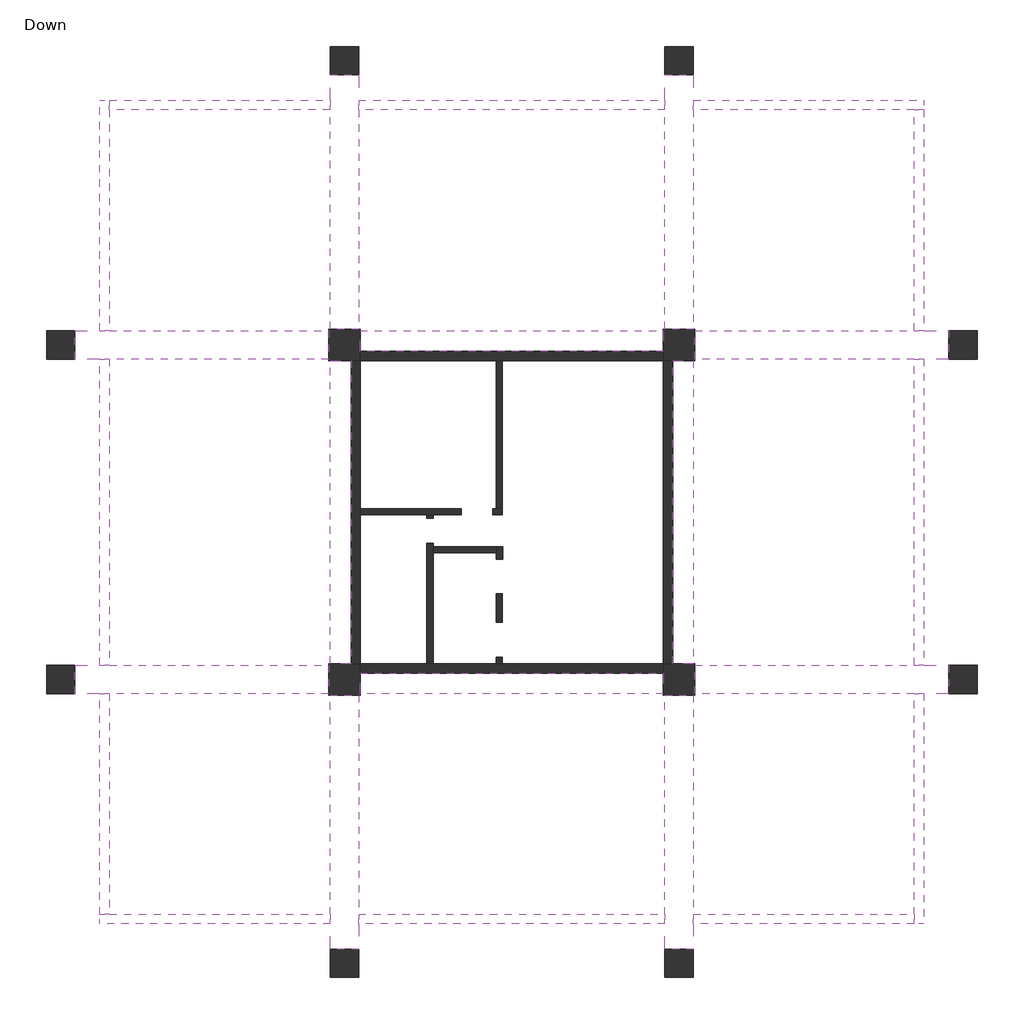
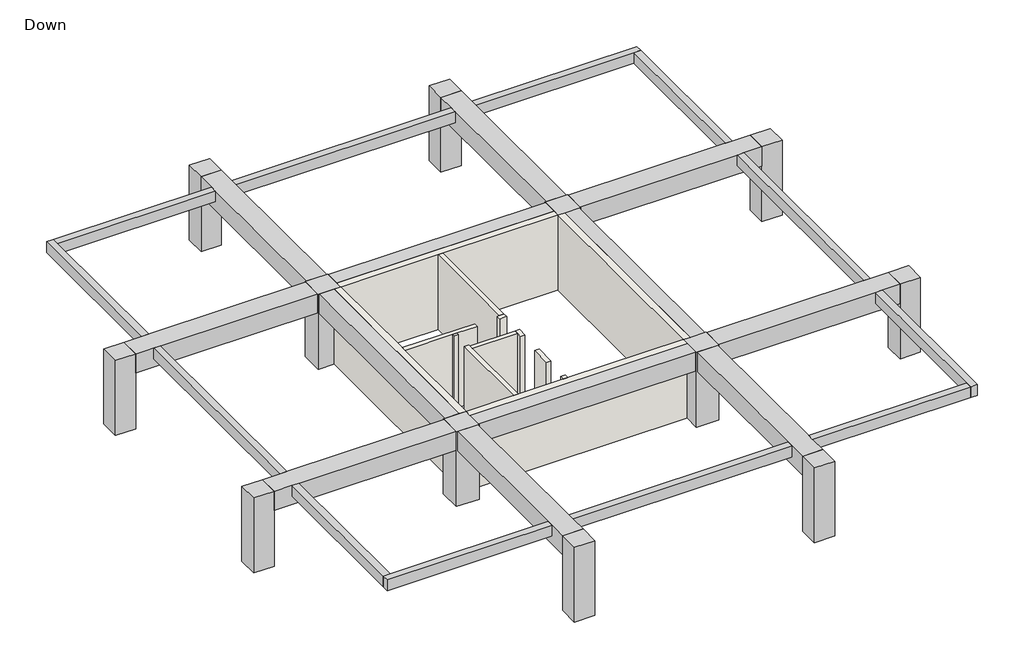
# One storey: 24 beams, 13 walls, 12 columns.
"""IFC4 building model written with IfcOpenShell, lengths in millimetres."""

import ifcopenshell
import ifcopenshell.guid

model = None  # the IFC model being written
_history = None  # IfcOwnerHistory: only IFC2X3 demands one
_inside = {}  # id of a spatial element -> (the spatial element, [elements in it])
_under = {}  # id of a project, library or spatial element -> (it, [spatial elements below it])
_declared = {}  # id of a project -> (the project, [libraries it declares])
_typed = {}  # id of a type object -> (the type object, [elements of that type])
_made_of = {}  # id of a material, layer set ... -> (it, [elements and type objects made of it])


def new_model(schema):
    """Start an empty IFC model of exactly this schema.

    Asked for "IFC4X3", IfcOpenShell would pick the latest addendum, in which some entities
    have other attributes; the version numbers below select the first issue.
    IFC2X3 requires an IfcOwnerHistory on every rooted entity: one is made here for all.
    """
    global model, _history
    if schema == "IFC4X3":
        model = ifcopenshell.file(schema_version=(4, 3, 0, 0))
    else:
        model = ifcopenshell.file(schema=schema)
    _inside.clear()
    _under.clear()
    _declared.clear()
    _typed.clear()
    _made_of.clear()
    _history = None
    if model.schema == "IFC2X3":
        org = make("IfcOrganization", Name="unknown")
        user = make(
            "IfcPersonAndOrganization",
            ThePerson=make("IfcPerson", FamilyName="unknown"),
            TheOrganization=org,
        )
        app = make(
            "IfcApplication",
            ApplicationDeveloper=org,
            Version="unknown",
            ApplicationFullName="unknown",
            ApplicationIdentifier="unknown",
        )
        _history = make(
            "IfcOwnerHistory",
            OwningUser=user,
            OwningApplication=app,
            ChangeAction="ADDED",
            CreationDate=0,
        )
    return model


def make(cls, **values):
    """One entity of the class cls with the attributes given. An attribute that is None is left unset."""
    return model.create_entity(
        cls, **{name: value for name, value in values.items() if value is not None}
    )


def rooted(cls, **values):
    """An entity with a GlobalId (a new one), such as an element, a storey or a relation."""
    return make(cls, GlobalId=ifcopenshell.guid.new(), OwnerHistory=_history, **values)


def si_unit(unit_type, name, prefix=None):
    """IfcSIUnit, for example si_unit("LENGTHUNIT", "METRE", prefix="MILLI")."""
    return make("IfcSIUnit", UnitType=unit_type, Prefix=prefix, Name=name)


def assignment(units):
    """IfcUnitAssignment: the units of a project."""
    return None if units is None else make("IfcUnitAssignment", Units=units)


def point(xyz):
    """IfcCartesianPoint."""
    return None if xyz is None else make("IfcCartesianPoint", Coordinates=xyz)


def direction(xyz):
    """IfcDirection."""
    return None if xyz is None else make("IfcDirection", DirectionRatios=xyz)


def frame(location, z_axis=None, x_axis=None):
    """IfcAxis2Placement3D, a coordinate frame: its origin and axes. An axis left out is left unset."""
    return make(
        "IfcAxis2Placement3D",
        Location=point(location),
        Axis=direction(z_axis),
        RefDirection=direction(x_axis),
    )


def origin():
    """The frame at (0, 0, 0) with its axes left unset."""
    return frame((0.0, 0.0, 0.0))


def origin_with_axes():
    """The frame at (0, 0, 0) with the z axis (0, 0, 1) and the x axis (1, 0, 0) written out."""
    return frame((0.0, 0.0, 0.0), z_axis=(0.0, 0.0, 1.0), x_axis=(1.0, 0.0, 0.0))


def place(relative_to, where):
    """IfcLocalPlacement: puts the frame where relative to a parent placement (None: the world)."""
    return make(
        "IfcLocalPlacement", PlacementRelTo=relative_to, RelativePlacement=where
    )


def context(
    kind, dimensions, precision=None, world=None, true_north=None, identifier=None
):
    """IfcGeometricRepresentationContext, for example the 3D "Model" context."""
    return make(
        "IfcGeometricRepresentationContext",
        ContextIdentifier=identifier,
        ContextType=kind,
        CoordinateSpaceDimension=dimensions,
        Precision=precision,
        WorldCoordinateSystem=world,
        TrueNorth=true_north,
    )


def project(units=None, contexts=None):
    """IfcProject with its units and contexts."""
    return rooted(
        "IfcProject",
        Name="project",
        RepresentationContexts=contexts,
        UnitsInContext=assignment(units),
    )


def spatial(cls, under=None, at=None, **own):
    """A site, building, storey or space (cls), placed at a placement, below another one or the project."""
    s = rooted(cls, ObjectPlacement=at, **own)
    if under is not None:
        _under.setdefault(under.id(), (under, []))[1].append(s)
    return s


def polyline(points):
    """IfcPolyline through the points."""
    return make("IfcPolyline", Points=[point(p) for p in points])


def outline(outer, holes=None, kind="AREA"):
    """IfcArbitraryClosedProfileDef: a profile drawn as a closed curve; with holes, ...WithVoids."""
    if holes is None:
        return make("IfcArbitraryClosedProfileDef", ProfileType=kind, OuterCurve=outer)
    return make(
        "IfcArbitraryProfileDefWithVoids",
        ProfileType=kind,
        OuterCurve=outer,
        InnerCurves=holes,
    )


def extrude(swept, where, along, depth):
    """IfcExtrudedAreaSolid: the profile swept, set in the frame where, extruded along a direction by depth."""
    return make(
        "IfcExtrudedAreaSolid",
        SweptArea=swept,
        Position=where,
        ExtrudedDirection=direction(along),
        Depth=depth,
    )


def faces_of(points, faces, orient=None, outer=None):
    """IfcFace entities. A face is a list of loops; a loop is a list of indices into points, from 0.

    orient and outer hold one flag for each loop. By default every Orientation is true, the
    first loop of a face is its IfcFaceOuterBound and the others are IfcFaceBound.
    """
    made = []
    for i, loops in enumerate(faces):
        bounds = []
        for j, loop in enumerate(loops):
            is_outer = j == 0 if outer is None else outer[i][j]
            bounds.append(
                make(
                    "IfcFaceOuterBound" if is_outer else "IfcFaceBound",
                    Bound=make("IfcPolyLoop", Polygon=[points[k] for k in loop]),
                    Orientation=True if orient is None else orient[i][j],
                )
            )
        made.append(make("IfcFace", Bounds=bounds))
    return made


def faceted_brep(points, faces, orient=None, outer=None, voids=None):
    """IfcFacetedBrep: a solid bounded by flat faces; with voids (closed shells), ...WithVoids."""
    shared = [point(p) for p in points]
    hull = make("IfcClosedShell", CfsFaces=faces_of(shared, faces, orient, outer))
    if voids is None:
        return make("IfcFacetedBrep", Outer=hull)
    return make(
        "IfcFacetedBrepWithVoids",
        Outer=hull,
        Voids=[
            make(cls, CfsFaces=faces_of(shared, fs, o, b)) for cls, fs, o, b in voids
        ],
    )


def shape(context_of_items, identifier, shape_type, items):
    """IfcShapeRepresentation: the items that make up one representation, for example the "Body"."""
    return make(
        "IfcShapeRepresentation",
        ContextOfItems=context_of_items,
        RepresentationIdentifier=identifier,
        RepresentationType=shape_type,
        Items=items,
    )


def made_of(thing, what):
    """Note that an element or type object is made of a material, layer set ...; save() writes the relation."""
    if what is not None:
        _made_of.setdefault(what.id(), (what, []))[1].append(thing)
    return thing


def element(
    cls,
    number,
    at=None,
    inside=None,
    cuts=None,
    type_object=None,
    material=None,
    context=None,
    identifier="Body",
    shape_type=None,
    held_by="IfcProductDefinitionShape",
    body=None,
    shapes=None,
    **own,
):
    """One element of the class cls, such as IfcWall. Its Tag is "e" and its number.

    at: its placement. inside: the storey or other place that contains it. cuts: it is an
    opening in that element (IfcRelVoidsElement). A single representation is given by context,
    identifier, shape_type and body (its items); several are given by shapes. held_by: the class
    of the entity that holds the representations. save() writes the other relations.
    """
    e = rooted(cls, Tag="e%d" % number, ObjectPlacement=at, **own)
    if body is not None:
        shapes = [shape(context, identifier, shape_type, body)]
    if shapes is not None:
        e.Representation = make(held_by, Representations=shapes)
    if inside is not None:
        _inside.setdefault(inside.id(), (inside, []))[1].append(e)
    if cuts is not None:
        rooted(
            "IfcRelVoidsElement", RelatingBuildingElement=cuts, RelatedOpeningElement=e
        )
    if type_object is not None:
        _typed.setdefault(type_object.id(), (type_object, []))[1].append(e)
    return made_of(e, material)


def aggregate(whole, parts):
    """IfcRelAggregates: a whole, such as a stair, and the parts it consists of."""
    return rooted("IfcRelAggregates", RelatingObject=whole, RelatedObjects=parts)


def save(model, path):
    """Write the relations noted so far, then the file.

    IfcRelAggregates (storeys below a building ...), IfcRelContainedInSpatialStructure (elements
    in a storey), IfcRelDefinesByType, IfcRelAssociatesMaterial and IfcRelDeclares: one each for
    every whole, place, type object, material and project.
    """
    for whole, parts in _under.values():
        aggregate(whole, parts)
    for where, things in _inside.values():
        rooted(
            "IfcRelContainedInSpatialStructure",
            RelatedElements=things,
            RelatingStructure=where,
        )
    for kind, things in _typed.values():
        rooted("IfcRelDefinesByType", RelatedObjects=things, RelatingType=kind)
    for what, things in _made_of.values():
        rooted("IfcRelAssociatesMaterial", RelatedObjects=things, RelatingMaterial=what)
    for by, libraries in _declared.values():
        rooted("IfcRelDeclares", RelatingContext=by, RelatedDefinitions=libraries)
    model.write(path)


model = new_model("IFC4")

# Units and contexts
model_context = context("Model", 3, world=origin())
ifc_project = project(units=[si_unit("LENGTHUNIT", "METRE", prefix="MILLI")], contexts=[model_context])

# Site, building, storey
site = spatial("IfcSite", under=ifc_project)
building = spatial("IfcBuilding", under=site)
storey = spatial("IfcBuildingStorey", under=building, Name="Down", Elevation=0.0)

# Beams
placement = place(None, origin())
element("IfcBeam", 1, ObjectType="Concrete Rectengular Beam : 30/50", at=placement, inside=storey, context=model_context, shape_type="Brep", body=[
    faceted_brep([(-5980.9538985, 16952.588413, 3500.0), (-5980.9538985, 17252.588413, 3500.0), (-15690.3344173, 17252.588413, 3500.0), (-15690.3344173, 16952.588413, 3500.0), (-5980.9538985, 16952.588413, 3000.0), (-5980.9538985, 16952.588413, 3250.0), (-15690.3344173, 16952.588413, 3250.0), (-15690.3344173, 16952.588413, 3000.0), (-5980.9538985, 17252.588413, 3000.0), (-15690.3344173, 17252.588413, 3000.0)], [[[0, 1, 2, 3]], [[4, 5, 0, 3, 6, 7]], [[8, 4, 7, 9]], [[1, 8, 9, 2]], [[1, 0, 5, 4, 8]], [[3, 2, 9, 7, 6]]]),
])
element("IfcBeam", 2, ObjectType="Concrete Rectengular Beam : 30/50", at=placement, inside=storey, context=model_context, shape_type="Brep", body=[
    faceted_brep([(2219.0461015, 16952.588413, 3500.0), (2219.0461015, 17252.588413, 3500.0), (-5080.9538985, 17252.588413, 3500.0), (-5080.9538985, 16952.588413, 3500.0), (1919.0461015, 16952.588413, 3500.0), (2219.0461015, 16952.588413, 3000.0), (-5080.9538985, 16952.588413, 3250.0), (-5080.9538985, 16952.588413, 3000.0), (1919.0461015, 16952.588413, 3000.0), (2219.0461015, 17252.588413, 3000.0), (-5080.9538985, 17252.588413, 3000.0)], [[[0, 1, 2, 3, 4]], [[5, 0, 4, 3, 6, 7, 8]], [[9, 5, 8, 7, 10]], [[1, 9, 10, 2]], [[3, 2, 10, 7, 6]], [[1, 0, 5, 9]]]),
])
element("IfcBeam", 3, ObjectType="Concrete Rectengular Beam : 30/50", at=placement, inside=storey, context=model_context, shape_type="Brep", body=[
    faceted_brep([(2219.0461015, 16952.588413, 3500.0), (1919.0461015, 16952.588413, 3500.0), (1919.0461015, 9953.1817285, 3500.0), (2219.0461015, 9953.1817285, 3500.0), (1919.0461015, 16952.588413, 3250.0), (1919.0461015, 16952.588413, 3000.0), (1919.0461015, 9953.1817285, 3000.0), (1919.0461015, 9953.1817285, 3250.0), (2219.0461015, 16952.588413, 3000.0), (2219.0461015, 9953.1817285, 3000.0)], [[[0, 1, 2, 3]], [[1, 4, 5, 6, 7, 2]], [[5, 8, 9, 6]], [[8, 0, 3, 9]], [[1, 0, 8, 5, 4]], [[3, 2, 7, 6, 9]]]),
])
element("IfcBeam", 4, ObjectType="Concrete Rectengular Beam : 30/50", at=placement, inside=storey, context=model_context, shape_type="Brep", body=[
    faceted_brep([(2219.0461015, 9053.1817285, 3500.0), (1919.0461015, 9053.1817285, 3500.0), (1919.0461015, -648.2491126, 3500.0), (2219.0461015, -648.2491126, 3500.0), (1919.0461015, 9053.1817285, 3250.0), (1919.0461015, 9053.1817285, 3000.0), (1919.0461015, -648.2491126, 3000.0), (1919.0461015, -648.2491126, 3250.0), (2219.0461015, 9053.1817285, 3000.0), (2219.0461015, -648.2491126, 3000.0)], [[[0, 1, 2, 3]], [[1, 4, 5, 6, 7, 2]], [[5, 8, 9, 6]], [[8, 0, 3, 9]], [[1, 0, 8, 5, 4]], [[3, 2, 7, 6, 9]]]),
])
element("IfcBeam", 5, ObjectType="Concrete Rectengular Beam : 30/50", at=placement, inside=storey, context=model_context, shape_type="Brep", body=[
    faceted_brep([(1919.0461015, -8848.2491126, 3500.0), (2219.0461015, -8848.2491126, 3500.0), (2219.0461015, -1548.2491126, 3500.0), (1919.0461015, -1548.2491126, 3500.0), (1919.0461015, -8548.2491126, 3500.0), (1919.0461015, -8848.2491126, 3000.0), (1919.0461015, -1548.2491126, 3250.0), (1919.0461015, -1548.2491126, 3000.0), (1919.0461015, -8548.2491126, 3000.0), (2219.0461015, -8848.2491126, 3000.0), (2219.0461015, -1548.2491126, 3000.0)], [[[0, 1, 2, 3, 4]], [[5, 0, 4, 3, 6, 7, 8]], [[9, 5, 8, 7, 10]], [[1, 9, 10, 2]], [[3, 2, 10, 7, 6]], [[1, 0, 5, 9]]]),
])
element("IfcBeam", 6, ObjectType="Concrete Rectengular Beam : 30/50", at=placement, inside=storey, context=model_context, shape_type="Brep", body=[
    faceted_brep([(1919.0461015, -8848.2491126, 3500.0), (1919.0461015, -8548.2491126, 3500.0), (-5080.9538985, -8548.2491126, 3500.0), (-5080.9538985, -8848.2491126, 3500.0), (1919.0461015, -8548.2491126, 3250.0), (1919.0461015, -8548.2491126, 3000.0), (-5080.9538985, -8548.2491126, 3000.0), (-5080.9538985, -8548.2491126, 3250.0), (1919.0461015, -8848.2491126, 3000.0), (-5080.9538985, -8848.2491126, 3000.0)], [[[0, 1, 2, 3]], [[1, 4, 5, 6, 7, 2]], [[5, 8, 9, 6]], [[8, 0, 3, 9]], [[1, 0, 8, 5, 4]], [[3, 2, 7, 6, 9]]]),
])
element("IfcBeam", 7, ObjectType="Concrete Rectengular Beam : 30/50", at=placement, inside=storey, context=model_context, shape_type="Brep", body=[
    faceted_brep([(-15690.3344173, -8548.2491126, 3500.0), (-15690.3344173, -8848.2491126, 3500.0), (-5980.9538985, -8848.2491126, 3500.0), (-5980.9538985, -8548.2491126, 3500.0), (-15690.3344173, -8548.2491126, 3000.0), (-15690.3344173, -8548.2491126, 3250.0), (-5980.9538985, -8548.2491126, 3250.0), (-5980.9538985, -8548.2491126, 3000.0), (-15690.3344173, -8848.2491126, 3000.0), (-5980.9538985, -8848.2491126, 3000.0)], [[[0, 1, 2, 3]], [[4, 5, 0, 3, 6, 7]], [[8, 4, 7, 9]], [[1, 8, 9, 2]], [[1, 0, 5, 4, 8]], [[3, 2, 9, 7, 6]]]),
])
element("IfcBeam", 8, ObjectType="Concrete Rectengular Beam : 30/50", at=placement, inside=storey, context=model_context, shape_type="Brep", body=[
    faceted_brep([(-23890.3344173, -8548.2491126, 3500.0), (-23890.3344173, -8848.2491126, 3500.0), (-16590.3344173, -8848.2491126, 3500.0), (-16590.3344173, -8548.2491126, 3500.0), (-23590.3344173, -8548.2491126, 3500.0), (-23890.3344173, -8548.2491126, 3000.0), (-16590.3344173, -8548.2491126, 3250.0), (-16590.3344173, -8548.2491126, 3000.0), (-23590.3344173, -8548.2491126, 3000.0), (-23890.3344173, -8848.2491126, 3000.0), (-16590.3344173, -8848.2491126, 3000.0)], [[[0, 1, 2, 3, 4]], [[5, 0, 4, 3, 6, 7, 8]], [[9, 5, 8, 7, 10]], [[1, 9, 10, 2]], [[3, 2, 10, 7, 6]], [[1, 0, 5, 9]]]),
])
element("IfcBeam", 9, ObjectType="Concrete Rectengular Beam : 30/50", at=placement, inside=storey, context=model_context, shape_type="Brep", body=[
    faceted_brep([(-23890.3344173, -8548.2491126, 3500.0), (-23590.3344173, -8548.2491126, 3500.0), (-23590.3344173, -1548.2491126, 3500.0), (-23890.3344173, -1548.2491126, 3500.0), (-23590.3344173, -8548.2491126, 3250.0), (-23590.3344173, -8548.2491126, 3000.0), (-23590.3344173, -1548.2491126, 3000.0), (-23590.3344173, -1548.2491126, 3250.0), (-23890.3344173, -8548.2491126, 3000.0), (-23890.3344173, -1548.2491126, 3000.0)], [[[0, 1, 2, 3]], [[1, 4, 5, 6, 7, 2]], [[5, 8, 9, 6]], [[8, 0, 3, 9]], [[1, 0, 8, 5, 4]], [[3, 2, 7, 6, 9]]]),
])
element("IfcBeam", 10, ObjectType="Concrete Rectengular Beam : 30/50", at=placement, inside=storey, context=model_context, shape_type="Brep", body=[
    faceted_brep([(-23590.3344173, 9053.1817285, 3500.0), (-23890.3344173, 9053.1817285, 3500.0), (-23890.3344173, -648.2491126, 3500.0), (-23590.3344173, -648.2491126, 3500.0), (-23590.3344173, 9053.1817285, 3000.0), (-23590.3344173, 9053.1817285, 3250.0), (-23590.3344173, -648.2491126, 3250.0), (-23590.3344173, -648.2491126, 3000.0), (-23890.3344173, 9053.1817285, 3000.0), (-23890.3344173, -648.2491126, 3000.0)], [[[0, 1, 2, 3]], [[4, 5, 0, 3, 6, 7]], [[8, 4, 7, 9]], [[1, 8, 9, 2]], [[1, 0, 5, 4, 8]], [[3, 2, 9, 7, 6]]]),
])
element("IfcBeam", 11, ObjectType="Concrete Rectengular Beam : 30/50", at=placement, inside=storey, context=model_context, shape_type="Brep", body=[
    faceted_brep([(-23590.3344173, 17253.1817285, 3500.0), (-23890.3344173, 17253.1817285, 3500.0), (-23890.3344173, 9953.1817285, 3500.0), (-23590.3344173, 9953.1817285, 3500.0), (-23590.3344173, 16953.1817285, 3500.0), (-23590.3344173, 17253.1817285, 3000.0), (-23590.3344173, 9953.1817285, 3250.0), (-23590.3344173, 9953.1817285, 3000.0), (-23590.3344173, 16953.1817285, 3000.0), (-23890.3344173, 17253.1817285, 3000.0), (-23890.3344173, 9953.1817285, 3000.0)], [[[0, 1, 2, 3, 4]], [[5, 0, 4, 3, 6, 7, 8]], [[9, 5, 8, 7, 10]], [[1, 9, 10, 2]], [[3, 2, 10, 7, 6]], [[1, 0, 5, 9]]]),
])
element("IfcBeam", 12, ObjectType="Concrete Rectengular Beam : 30/50", at=placement, inside=storey, context=model_context, shape_type="Brep", body=[
    faceted_brep([(-23590.3344173, 17253.1817285, 3500.0), (-23590.3344173, 16953.1817285, 3500.0), (-16590.3344173, 16953.1817285, 3500.0), (-16590.3344173, 17253.1817285, 3500.0), (-23590.3344173, 16953.1817285, 3250.0), (-23590.3344173, 16953.1817285, 3000.0), (-16590.3344173, 16953.1817285, 3000.0), (-16590.3344173, 16953.1817285, 3250.0), (-23590.3344173, 17253.1817285, 3000.0), (-16590.3344173, 17253.1817285, 3000.0)], [[[0, 1, 2, 3]], [[1, 4, 5, 6, 7, 2]], [[5, 8, 9, 6]], [[8, 0, 3, 9]], [[1, 0, 8, 5, 4]], [[3, 2, 7, 6, 9]]]),
])
element("IfcBeam", 13, ObjectType="Concrete Rectengular Beam : 90/90", at=placement, inside=storey, context=model_context, shape_type="Brep", body=[
    faceted_brep([(3013.7426277, 9053.1817285, 3500.0), (3013.7426277, 9953.1817285, 3500.0), (2219.0461015, 9953.1817285, 3500.0), (1919.0461015, 9953.1817285, 3500.0), (-5030.9538985, 9953.1817285, 3500.0), (-5030.9538985, 9053.1817285, 3500.0), (1919.0461015, 9053.1817285, 3500.0), (2219.0461015, 9053.1817285, 3500.0), (3013.7426277, 9953.1817285, 2600.0), (-5030.9538985, 9953.1817285, 2600.0), (-5030.9538985, 9953.1817285, 3250.0), (3013.7426277, 9053.1817285, 2600.0), (-5030.9538985, 9053.1817285, 2600.0), (-5030.9538985, 9053.1817285, 3250.0)], [[[0, 1, 2, 3, 4, 5, 6, 7]], [[1, 8, 9, 10, 4, 3, 2]], [[8, 11, 12, 9]], [[11, 0, 7, 6, 5, 13, 12]], [[1, 0, 11, 8]], [[5, 4, 10, 9, 12, 13]]]),
])
element("IfcBeam", 14, ObjectType="Concrete Rectengular Beam : 90/90", at=placement, inside=storey, context=model_context, shape_type="Brep", body=[
    faceted_brep([(-6030.9538985, 9953.1817285, 3500.0), (-15640.3344173, 9953.1817285, 3500.0), (-15640.3344173, 9303.1817285, 3500.0), (-6030.9538985, 9303.1817285, 3500.0), (-15640.3344173, 9953.1817285, 2600.0), (-15640.3344173, 9953.1817285, 3250.0), (-6030.9538985, 9953.1817285, 3250.0), (-6030.9538985, 9953.1817285, 2600.0), (-6030.9538985, 9303.1817285, 2600.0), (-15640.3344173, 9303.1817285, 2600.0)], [[[0, 1, 2, 3]], [[4, 5, 1, 0, 6, 7]], [[4, 7, 8, 9]], [[1, 5, 4, 9, 2]], [[7, 6, 0, 3, 8]], [[3, 2, 9, 8]]]),
])
element("IfcBeam", 15, ObjectType="Concrete Rectengular Beam : 90/90", at=placement, inside=storey, context=model_context, shape_type="Brep", body=[
    faceted_brep([(-24681.3411297, 9953.1817285, 3500.0), (-24681.3411297, 9053.1817285, 3500.0), (-23890.3344173, 9053.1817285, 3500.0), (-23590.3344173, 9053.1817285, 3500.0), (-16640.3344173, 9053.1817285, 3500.0), (-16640.3344173, 9953.1817285, 3500.0), (-23590.3344173, 9953.1817285, 3500.0), (-23890.3344173, 9953.1817285, 3500.0), (-24681.3411297, 9953.1817285, 2600.0), (-16640.3344173, 9953.1817285, 3250.0), (-16640.3344173, 9953.1817285, 2600.0), (-24681.3411297, 9053.1817285, 2600.0), (-16640.3344173, 9053.1817285, 2600.0), (-16640.3344173, 9053.1817285, 3250.0)], [[[0, 1, 2, 3, 4, 5, 6, 7]], [[8, 0, 7, 6, 5, 9, 10]], [[11, 8, 10, 12]], [[1, 11, 12, 13, 4, 3, 2]], [[1, 0, 8, 11]], [[5, 4, 13, 12, 10, 9]]]),
])
element("IfcBeam", 16, ObjectType="Concrete Rectengular Beam : 90/90", at=placement, inside=storey, context=model_context, shape_type="Brep", body=[
    faceted_brep([(-5080.9538985, 18056.4963349, 3500.0), (-5980.9538985, 18056.4963349, 3500.0), (-5980.9538985, 17252.588413, 3500.0), (-5980.9538985, 16952.588413, 3500.0), (-5980.9538985, 10003.1817285, 3500.0), (-5080.9538985, 10003.1817285, 3500.0), (-5080.9538985, 16952.588413, 3500.0), (-5080.9538985, 17252.588413, 3500.0), (-5080.9538985, 18056.4963349, 2600.0), (-5080.9538985, 10003.1817285, 3250.0), (-5080.9538985, 10003.1817285, 2600.0), (-5980.9538985, 18056.4963349, 2600.0), (-5980.9538985, 10003.1817285, 2600.0), (-5980.9538985, 10003.1817285, 3250.0)], [[[0, 1, 2, 3, 4, 5, 6, 7]], [[8, 0, 7, 6, 5, 9, 10]], [[11, 8, 10, 12]], [[1, 11, 12, 13, 4, 3, 2]], [[1, 0, 8, 11]], [[5, 4, 13, 12, 10, 9]]]),
])
element("IfcBeam", 17, ObjectType="Concrete Rectengular Beam : 90/90", at=placement, inside=storey, context=model_context, shape_type="Brep", body=[
    faceted_brep([(-15690.3344173, 18056.4963349, 3500.0), (-16590.3344173, 18056.4963349, 3500.0), (-16590.3344173, 17253.1817285, 3500.0), (-16590.3344173, 16953.1817285, 3500.0), (-16590.3344173, 10003.1817285, 3500.0), (-15690.3344173, 10003.1817285, 3500.0), (-15690.3344173, 16952.588413, 3500.0), (-15690.3344173, 17252.588413, 3500.0), (-16590.3344173, 18056.4963349, 2600.0), (-16590.3344173, 10003.1817285, 2600.0), (-16590.3344173, 10003.1817285, 3250.0), (-15690.3344173, 18056.4963349, 2600.0), (-15690.3344173, 10003.1817285, 2600.0), (-15690.3344173, 10003.1817285, 3250.0)], [[[0, 1, 2, 3, 4, 5, 6, 7]], [[1, 8, 9, 10, 4, 3, 2]], [[8, 11, 12, 9]], [[11, 0, 7, 6, 5, 13, 12]], [[1, 0, 11, 8]], [[5, 4, 10, 9, 12, 13]]]),
])
element("IfcBeam", 18, ObjectType="Concrete Rectengular Beam : 90/90", at=placement, inside=storey, context=model_context, shape_type="Brep", body=[
    faceted_brep([(-24681.3411297, -648.2491126, 3500.0), (-24681.3411297, -1548.2491126, 3500.0), (-23890.3344173, -1548.2491126, 3500.0), (-23590.3344173, -1548.2491126, 3500.0), (-16640.3344173, -1548.2491126, 3500.0), (-16640.3344173, -648.2491126, 3500.0), (-23590.3344173, -648.2491126, 3500.0), (-23890.3344173, -648.2491126, 3500.0), (-24681.3411297, -1548.2491126, 2600.0), (-16640.3344173, -1548.2491126, 2600.0), (-16640.3344173, -1548.2491126, 3250.0), (-24681.3411297, -648.2491126, 2600.0), (-16640.3344173, -648.2491126, 2600.0), (-16640.3344173, -648.2491126, 3250.0)], [[[0, 1, 2, 3, 4, 5, 6, 7]], [[1, 8, 9, 10, 4, 3, 2]], [[8, 11, 12, 9]], [[11, 0, 7, 6, 5, 13, 12]], [[1, 0, 11, 8]], [[5, 4, 10, 9, 12, 13]]]),
])
element("IfcBeam", 19, ObjectType="Concrete Rectengular Beam : 90/90", at=placement, inside=storey, context=model_context, shape_type="Brep", body=[
    faceted_brep([(-16590.3344173, -9646.694756, 3500.0), (-15690.3344173, -9646.694756, 3500.0), (-15690.3344173, -8848.2491126, 3500.0), (-15690.3344173, -8548.2491126, 3500.0), (-15690.3344173, -1598.2491126, 3500.0), (-16590.3344173, -1598.2491126, 3500.0), (-16590.3344173, -8548.2491126, 3500.0), (-16590.3344173, -8848.2491126, 3500.0), (-16590.3344173, -9646.694756, 2600.0), (-16590.3344173, -1598.2491126, 3250.0), (-16590.3344173, -1598.2491126, 2600.0), (-15690.3344173, -9646.694756, 2600.0), (-15690.3344173, -1598.2491126, 2600.0), (-15690.3344173, -1598.2491126, 3250.0)], [[[0, 1, 2, 3, 4, 5, 6, 7]], [[8, 0, 7, 6, 5, 9, 10]], [[11, 8, 10, 12]], [[1, 11, 12, 13, 4, 3, 2]], [[1, 0, 8, 11]], [[5, 4, 13, 12, 10, 9]]]),
])
element("IfcBeam", 20, ObjectType="Concrete Rectengular Beam : 90/90", at=placement, inside=storey, context=model_context, shape_type="Brep", body=[
    faceted_brep([(-5980.9538985, -9646.694756, 3500.0), (-5080.9538985, -9646.694756, 3500.0), (-5080.9538985, -8848.2491126, 3500.0), (-5080.9538985, -8548.2491126, 3500.0), (-5080.9538985, -1598.2491126, 3500.0), (-5980.9538985, -1598.2491126, 3500.0), (-5980.9538985, -8548.2491126, 3500.0), (-5980.9538985, -8848.2491126, 3500.0), (-5980.9538985, -9646.694756, 2600.0), (-5980.9538985, -1598.2491126, 3250.0), (-5980.9538985, -1598.2491126, 2600.0), (-5080.9538985, -9646.694756, 2600.0), (-5080.9538985, -1598.2491126, 2600.0), (-5080.9538985, -1598.2491126, 3250.0)], [[[0, 1, 2, 3, 4, 5, 6, 7]], [[8, 0, 7, 6, 5, 9, 10]], [[11, 8, 10, 12]], [[1, 11, 12, 13, 4, 3, 2]], [[1, 0, 8, 11]], [[5, 4, 13, 12, 10, 9]]]),
])
element("IfcBeam", 21, ObjectType="Concrete Rectengular Beam : 90/90", at=placement, inside=storey, context=model_context, shape_type="Brep", body=[
    faceted_brep([(3013.7426277, -1548.2491126, 3500.0), (3013.7426277, -648.2491126, 3500.0), (2219.0461015, -648.2491126, 3500.0), (1919.0461015, -648.2491126, 3500.0), (-5030.9538985, -648.2491126, 3500.0), (-5030.9538985, -1548.2491126, 3500.0), (1919.0461015, -1548.2491126, 3500.0), (2219.0461015, -1548.2491126, 3500.0), (3013.7426277, -648.2491126, 2600.0), (-5030.9538985, -648.2491126, 2600.0), (-5030.9538985, -648.2491126, 3250.0), (3013.7426277, -1548.2491126, 2600.0), (-5030.9538985, -1548.2491126, 2600.0), (-5030.9538985, -1548.2491126, 3250.0)], [[[0, 1, 2, 3, 4, 5, 6, 7]], [[1, 8, 9, 10, 4, 3, 2]], [[8, 11, 12, 9]], [[11, 0, 7, 6, 5, 13, 12]], [[1, 0, 11, 8]], [[5, 4, 10, 9, 12, 13]]]),
])
element("IfcBeam", 22, ObjectType="Concrete Rectengular Beam : 90/90", at=placement, inside=storey, context=model_context, shape_type="Brep", body=[
    faceted_brep([(-5080.9538985, -598.2491126, 3500.0), (-5080.9538985, 9003.1817285, 3500.0), (-5730.9538985, 9003.1817285, 3500.0), (-5730.9538985, -598.2491126, 3500.0), (-5080.9538985, 9003.1817285, 2600.0), (-5080.9538985, -598.2491126, 2600.0), (-5730.9538985, -598.2491126, 2600.0), (-5730.9538985, 9003.1817285, 2600.0), (-5080.9538985, 9003.1817285, 3250.0), (-5080.9538985, -598.2491126, 3250.0)], [[[0, 1, 2, 3]], [[4, 5, 6, 7]], [[4, 8, 1, 0, 9, 5]], [[1, 8, 4, 7, 2]], [[5, 9, 0, 3, 6]], [[3, 2, 7, 6]]]),
])
element("IfcBeam", 23, ObjectType="Concrete Rectengular Beam : 90/90", at=placement, inside=storey, context=model_context, shape_type="Brep", body=[
    faceted_brep([(-16590.3344173, 9003.1817285, 3500.0), (-16590.3344173, -598.2491126, 3500.0), (-15931.2318689, -598.2491126, 3500.0), (-15931.2318689, 9003.1817285, 3500.0), (-16590.3344173, -598.2491126, 2600.0), (-16590.3344173, 9003.1817285, 2600.0), (-15931.2318689, 9003.1817285, 2600.0), (-15931.2318689, -598.2491126, 2600.0), (-16590.3344173, 9003.1817285, 3250.0), (-16590.3344173, -598.2491126, 3250.0)], [[[0, 1, 2, 3]], [[4, 5, 6, 7]], [[0, 8, 5, 4, 9, 1]], [[5, 8, 0, 3, 6]], [[1, 9, 4, 7, 2]], [[3, 2, 7, 6]]]),
])
element("IfcBeam", 24, ObjectType="Concrete Rectengular Beam : 90/90", at=placement, inside=storey, context=model_context, shape_type="Brep", body=[
    faceted_brep([(-15640.3344173, -1548.2491126, 3500.0), (-6030.9538985, -1548.2491126, 3500.0), (-6030.9538985, -898.2491126, 3500.0), (-15640.3344173, -898.2491126, 3500.0), (-6030.9538985, -1548.2491126, 2600.0), (-6030.9538985, -1548.2491126, 3250.0), (-15640.3344173, -1548.2491126, 3250.0), (-15640.3344173, -1548.2491126, 2600.0), (-15640.3344173, -898.2491126, 2600.0), (-6030.9538985, -898.2491126, 2600.0)], [[[0, 1, 2, 3]], [[4, 5, 1, 0, 6, 7]], [[4, 7, 8, 9]], [[1, 5, 4, 9, 2]], [[7, 6, 0, 3, 8]], [[3, 2, 9, 8]]]),
])

# Columns
element("IfcColumn", 25, ObjectType="Concrete Rectengular Column : 100/100", at=placement, inside=storey, context=model_context, shape_type="Brep", body=[
    faceted_brep([(-15640.3344173, 10003.1817285, 0.0), (-15640.3344173, 9303.1817285, 0.0), (-15640.3344173, 9003.1817285, 0.0), (-15931.2318689, 9003.1817285, 0.0), (-16640.3344173, 9003.1817285, 0.0), (-16640.3344173, 10003.1817285, 0.0), (-15640.3344173, 10003.1817285, 3500.0), (-15640.3344173, 9953.1817285, 3500.0), (-15640.3344173, 9303.1817285, 3500.0), (-15640.3344173, 9003.1817285, 3500.0), (-15640.3344173, 10003.1817285, 3250.0), (-15931.2318689, 9003.1817285, 3500.0), (-16590.3344173, 9003.1817285, 3500.0), (-16640.3344173, 9003.1817285, 3500.0), (-16640.3344173, 9003.1817285, 3250.0), (-16640.3344173, 9053.1817285, 3500.0), (-16640.3344173, 9953.1817285, 3500.0), (-16640.3344173, 10003.1817285, 3500.0), (-16640.3344173, 10003.1817285, 3250.0), (-16590.3344173, 10003.1817285, 3500.0), (-15690.3344173, 10003.1817285, 3500.0)], [[[0, 1, 2, 3, 4, 5]], [[6, 7, 8, 9, 2, 1, 0, 10]], [[9, 11, 12, 13, 14, 4, 3, 2]], [[13, 15, 16, 17, 18, 5, 4, 14]], [[17, 19, 20, 6, 10, 0, 5, 18]], [[6, 20, 19, 17, 16, 15, 13, 12, 11, 9, 8, 7]]]),
])
element("IfcColumn", 26, ObjectType="Concrete Rectengular Column : 100/100", at=placement, inside=storey, context=model_context, shape_type="Brep", body=[
    faceted_brep([(-5030.9538985, 10003.1817285, 0.0), (-5030.9538985, 9003.1817285, 0.0), (-5730.9538985, 9003.1817285, 0.0), (-6030.9538985, 9003.1817285, 0.0), (-6030.9538985, 9303.1817285, 0.0), (-6030.9538985, 10003.1817285, 0.0), (-5030.9538985, 10003.1817285, 3500.0), (-5030.9538985, 9953.1817285, 3500.0), (-5030.9538985, 9053.1817285, 3500.0), (-5030.9538985, 9003.1817285, 3500.0), (-5030.9538985, 9003.1817285, 3250.0), (-5030.9538985, 10003.1817285, 3250.0), (-5080.9538985, 9003.1817285, 3500.0), (-5730.9538985, 9003.1817285, 3500.0), (-6030.9538985, 9003.1817285, 3500.0), (-6030.9538985, 9303.1817285, 3500.0), (-6030.9538985, 9953.1817285, 3500.0), (-6030.9538985, 10003.1817285, 3500.0), (-6030.9538985, 10003.1817285, 3250.0), (-5980.9538985, 10003.1817285, 3500.0), (-5080.9538985, 10003.1817285, 3500.0)], [[[0, 1, 2, 3, 4, 5]], [[6, 7, 8, 9, 10, 1, 0, 11]], [[9, 12, 13, 14, 3, 2, 1, 10]], [[14, 15, 16, 17, 18, 5, 4, 3]], [[17, 19, 20, 6, 11, 0, 5, 18]], [[6, 20, 19, 17, 16, 15, 14, 13, 12, 9, 8, 7]]]),
])
element("IfcColumn", 27, ObjectType="Concrete Rectengular Column : 100/100", at=placement, inside=storey, context=model_context, shape_type="Brep", body=[
    faceted_brep([(-5030.9538985, -598.2491126, 0.0), (-5030.9538985, -1598.2491126, 0.0), (-6030.9538985, -1598.2491126, 0.0), (-6030.9538985, -898.2491126, 0.0), (-6030.9538985, -598.2491126, 0.0), (-5730.9538985, -598.2491126, 0.0), (-5030.9538985, -598.2491126, 3500.0), (-5030.9538985, -648.2491126, 3500.0), (-5030.9538985, -1548.2491126, 3500.0), (-5030.9538985, -1598.2491126, 3500.0), (-5030.9538985, -1598.2491126, 3250.0), (-5030.9538985, -598.2491126, 3250.0), (-5080.9538985, -1598.2491126, 3500.0), (-5980.9538985, -1598.2491126, 3500.0), (-6030.9538985, -1598.2491126, 3500.0), (-6030.9538985, -1598.2491126, 3250.0), (-6030.9538985, -1548.2491126, 3500.0), (-6030.9538985, -898.2491126, 3500.0), (-6030.9538985, -598.2491126, 3500.0), (-5730.9538985, -598.2491126, 3500.0), (-5080.9538985, -598.2491126, 3500.0)], [[[0, 1, 2, 3, 4, 5]], [[6, 7, 8, 9, 10, 1, 0, 11]], [[9, 12, 13, 14, 15, 2, 1, 10]], [[14, 16, 17, 18, 4, 3, 2, 15]], [[18, 19, 20, 6, 11, 0, 5, 4]], [[6, 20, 19, 18, 17, 16, 14, 13, 12, 9, 8, 7]]]),
])
element("IfcColumn", 28, ObjectType="Concrete Rectengular Column : 100/100", at=placement, inside=storey, context=model_context, shape_type="Brep", body=[
    faceted_brep([(-15640.3344173, -598.2491126, 0.0), (-15640.3344173, -898.2491126, 0.0), (-15640.3344173, -1598.2491126, 0.0), (-16640.3344173, -1598.2491126, 0.0), (-16640.3344173, -598.2491126, 0.0), (-15931.2318689, -598.2491126, 0.0), (-15640.3344173, -598.2491126, 3500.0), (-15640.3344173, -898.2491126, 3500.0), (-15640.3344173, -1548.2491126, 3500.0), (-15640.3344173, -1598.2491126, 3500.0), (-15640.3344173, -1598.2491126, 3250.0), (-15690.3344173, -1598.2491126, 3500.0), (-16590.3344173, -1598.2491126, 3500.0), (-16640.3344173, -1598.2491126, 3500.0), (-16640.3344173, -1598.2491126, 3250.0), (-16640.3344173, -1548.2491126, 3500.0), (-16640.3344173, -648.2491126, 3500.0), (-16640.3344173, -598.2491126, 3500.0), (-16640.3344173, -598.2491126, 3250.0), (-16590.3344173, -598.2491126, 3500.0), (-15931.2318689, -598.2491126, 3500.0)], [[[0, 1, 2, 3, 4, 5]], [[6, 7, 8, 9, 10, 2, 1, 0]], [[9, 11, 12, 13, 14, 3, 2, 10]], [[13, 15, 16, 17, 18, 4, 3, 14]], [[17, 19, 20, 6, 0, 5, 4, 18]], [[6, 20, 19, 17, 16, 15, 13, 12, 11, 9, 8, 7]]]),
])
element("IfcColumn", 29, ObjectType="Concrete Rectengular Column : 90/90", at=placement, inside=storey, context=model_context, shape_type="SweptSolid", body=[
    extrude(outline(polyline([(-24681.3411297, -648.2491126), (-24681.3411297, -1548.2491126), (-25581.3411297, -1548.2491126), (-25581.3411297, -648.2491126), (-24681.3411297, -648.2491126)])), origin_with_axes(), (0.0, 0.0, 1.0), 3500.0),
])
element("IfcColumn", 30, ObjectType="Concrete Rectengular Column : 90/90", at=placement, inside=storey, context=model_context, shape_type="SweptSolid", body=[
    extrude(outline(polyline([(-24681.3411297, 9953.1817285), (-24681.3411297, 9053.1817285), (-25581.3411297, 9053.1817285), (-25581.3411297, 9953.1817285), (-24681.3411297, 9953.1817285)])), origin_with_axes(), (0.0, 0.0, 1.0), 3500.0),
])
element("IfcColumn", 31, ObjectType="Concrete Rectengular Column : 90/90", at=placement, inside=storey, context=model_context, shape_type="SweptSolid", body=[
    extrude(outline(polyline([(-15690.3344173, -9646.694756), (-15690.3344173, -10546.694756), (-16590.3344173, -10546.694756), (-16590.3344173, -9646.694756), (-15690.3344173, -9646.694756)])), origin_with_axes(), (0.0, 0.0, 1.0), 3500.0),
])
element("IfcColumn", 32, ObjectType="Concrete Rectengular Column : 90/90", at=placement, inside=storey, context=model_context, shape_type="SweptSolid", body=[
    extrude(outline(polyline([(-5080.9538985, -9646.694756), (-5080.9538985, -10546.694756), (-5980.9538985, -10546.694756), (-5980.9538985, -9646.694756), (-5080.9538985, -9646.694756)])), origin_with_axes(), (0.0, 0.0, 1.0), 3500.0),
])
element("IfcColumn", 33, ObjectType="Concrete Rectengular Column : 90/90", at=placement, inside=storey, context=model_context, shape_type="SweptSolid", body=[
    extrude(outline(polyline([(3913.7426277, -648.2491126), (3913.7426277, -1548.2491126), (3013.7426277, -1548.2491126), (3013.7426277, -648.2491126), (3913.7426277, -648.2491126)])), origin_with_axes(), (0.0, 0.0, 1.0), 3500.0),
])
element("IfcColumn", 34, ObjectType="Concrete Rectengular Column : 90/90", at=placement, inside=storey, context=model_context, shape_type="SweptSolid", body=[
    extrude(outline(polyline([(3913.7426277, 9953.1817285), (3913.7426277, 9053.1817285), (3013.7426277, 9053.1817285), (3013.7426277, 9953.1817285), (3913.7426277, 9953.1817285)])), origin_with_axes(), (0.0, 0.0, 1.0), 3500.0),
])
element("IfcColumn", 35, ObjectType="Concrete Rectengular Column : 90/90", at=placement, inside=storey, context=model_context, shape_type="SweptSolid", body=[
    extrude(outline(polyline([(-5080.9538985, 18956.4963349), (-5080.9538985, 18056.4963349), (-5980.9538985, 18056.4963349), (-5980.9538985, 18956.4963349), (-5080.9538985, 18956.4963349)])), origin_with_axes(), (0.0, 0.0, 1.0), 3500.0),
])
element("IfcColumn", 36, ObjectType="Concrete Rectengular Column : 90/90", at=placement, inside=storey, context=model_context, shape_type="SweptSolid", body=[
    extrude(outline(polyline([(-15690.3344173, 18956.4963349), (-15690.3344173, 18056.4963349), (-16590.3344173, 18056.4963349), (-16590.3344173, 18956.4963349), (-15690.3344173, 18956.4963349)])), origin_with_axes(), (0.0, 0.0, 1.0), 3500.0),
])

# Walls
element("IfcWall", 37, ObjectType="20", at=placement, inside=storey, context=model_context, shape_type="Brep", body=[
    faceted_brep([(-15631.2318689, 4110.3323713, 0.0), (-13530.6176456, 4110.3323713, 0.0), (-13330.6176456, 4110.3323713, 0.0), (-12431.1134644, 4110.3323713, 0.0), (-12431.1134644, 4110.3323713, 3250.0), (-12431.1134644, 4110.3323713, 3500.0), (-13330.6176456, 4110.3323713, 3500.0), (-13530.6176456, 4110.3323713, 3500.0), (-15631.2318689, 4110.3323713, 3500.0), (-15631.2318689, 4310.3323713, 0.0), (-15631.2318689, 4310.3323713, 3250.0), (-15631.2318689, 4310.3323713, 3500.0), (-12431.1134644, 4310.3323713, 3500.0), (-12431.1134644, 4310.3323713, 3250.0), (-12431.1134644, 4310.3323713, 0.0)], [[[0, 1, 2, 3, 4, 5, 6, 7, 8]], [[9, 10, 11, 12, 13, 14]], [[3, 2, 1, 0, 9, 14]], [[5, 4, 3, 14, 13, 12]], [[8, 7, 6, 5, 12, 11]], [[0, 8, 11, 10, 9]]]),
])
element("IfcWall", 38, ObjectType="20", at=placement, inside=storey, context=model_context, shape_type="Brep", body=[
    faceted_brep([(-13530.6176456, 4110.3323713, 0.0), (-13530.6176456, 4008.7413108, 0.0), (-13530.6176456, 4008.7413108, 3250.0), (-13530.6176456, 4008.7413108, 3500.0), (-13530.6176456, 4110.3323713, 3500.0), (-13330.6176456, 4110.3323713, 0.0), (-13330.6176456, 4110.3323713, 3250.0), (-13330.6176456, 4110.3323713, 3500.0), (-13330.6176456, 4008.7413108, 3500.0), (-13330.6176456, 4008.7413108, 3250.0), (-13330.6176456, 4008.7413108, 0.0)], [[[0, 1, 2, 3, 4]], [[5, 6, 7, 8, 9, 10]], [[1, 0, 5, 10]], [[3, 2, 1, 10, 9, 8]], [[4, 3, 8, 7]], [[0, 4, 7, 6, 5]]]),
])
element("IfcWall", 39, ObjectType="20", at=placement, inside=storey, context=model_context, shape_type="Brep", body=[
    faceted_brep([(-11432.1347032, 4110.3323713, 0.0), (-11131.5944827, 4110.3323713, 0.0), (-11131.5944827, 4110.3323713, 3250.0), (-11131.5944827, 4110.3323713, 3500.0), (-11136.5944827, 4110.3323713, 3500.0), (-11432.1347032, 4110.3323713, 3500.0), (-11432.1347032, 4110.3323713, 3250.0), (-11432.1347032, 4310.3323713, 0.0), (-11432.1347032, 4310.3323713, 3250.0), (-11432.1347032, 4310.3323713, 3500.0), (-11331.5944827, 4310.3323713, 3500.0), (-11131.5944827, 4310.3323713, 3500.0), (-11131.5944827, 4310.3323713, 0.0), (-11331.5944827, 4310.3323713, 0.0)], [[[0, 1, 2, 3, 4, 5, 6]], [[7, 8, 9, 10, 11, 12, 13]], [[1, 0, 7, 13, 12]], [[5, 4, 3, 11, 10, 9]], [[0, 6, 5, 9, 8, 7]], [[3, 2, 1, 12, 11]]]),
])
element("IfcWall", 40, ObjectType="20", at=placement, inside=storey, context=model_context, shape_type="Brep", body=[
    faceted_brep([(-11131.5944827, 4310.3323713, 0.0), (-11131.5944827, 9003.1817285, 0.0), (-11131.5944827, 9003.1817285, 3250.0), (-11131.5944827, 9003.1817285, 3500.0), (-11131.5944827, 4310.3323713, 3500.0), (-11331.5944827, 4310.3323713, 0.0), (-11331.5944827, 4310.3323713, 3250.0), (-11331.5944827, 4310.3323713, 3500.0), (-11331.5944827, 9003.1817285, 3500.0), (-11331.5944827, 9003.1817285, 3250.0), (-11331.5944827, 9003.1817285, 0.0)], [[[0, 1, 2, 3, 4]], [[5, 6, 7, 8, 9, 10]], [[1, 0, 5, 10]], [[4, 3, 8, 7]], [[0, 4, 7, 6, 5]], [[3, 2, 1, 10, 9, 8]]]),
])
element("IfcWall", 41, ObjectType="20", at=placement, inside=storey, context=model_context, shape_type="Brep", body=[
    faceted_brep([(-13530.6176456, 3208.7117097, 0.0), (-13530.6176456, -598.2491126, 0.0), (-13530.6176456, -598.2491126, 3500.0), (-13530.6176456, 3208.7117097, 3500.0), (-13530.6176456, 3208.7117097, 3250.0), (-13330.6176456, 3208.7117097, 0.0), (-13330.6176456, 3208.7117097, 3250.0), (-13330.6176456, 3208.7117097, 3500.0), (-13330.6176456, 3109.2371297, 3500.0), (-13330.6176456, 2909.2371297, 3500.0), (-13330.6176456, -598.2491126, 3500.0), (-13330.6176456, -598.2491126, 0.0), (-13330.6176456, 2909.2371297, 0.0), (-13330.6176456, 3109.2371297, 0.0)], [[[0, 1, 2, 3, 4]], [[5, 6, 7, 8, 9, 10, 11, 12, 13]], [[1, 0, 5, 13, 12, 11]], [[3, 2, 10, 9, 8, 7]], [[0, 4, 3, 7, 6, 5]], [[2, 1, 11, 10]]]),
])
element("IfcWall", 42, ObjectType="20", at=placement, inside=storey, context=model_context, shape_type="Brep", body=[
    faceted_brep([(-13330.6176456, 2909.2371297, 0.0), (-11330.6176456, 2909.2371297, 0.0), (-11330.6176456, 2909.2371297, 3500.0), (-13330.6176456, 2909.2371297, 3500.0), (-13330.6176456, 3109.2371297, 0.0), (-13330.6176456, 3109.2371297, 3250.0), (-13330.6176456, 3109.2371297, 3500.0), (-11330.6176456, 3109.2371297, 3500.0), (-11330.6176456, 3109.2371297, 0.0)], [[[0, 1, 2, 3]], [[4, 5, 6, 7, 8]], [[1, 0, 4, 8]], [[3, 2, 7, 6]], [[0, 3, 6, 5, 4]], [[2, 1, 8, 7]]]),
])
element("IfcWall", 43, ObjectType="20", at=placement, inside=storey, context=model_context, shape_type="Brep", body=[
    faceted_brep([(-11330.6176456, 3109.2371297, 0.0), (-11330.6176456, 2909.2371297, 0.0), (-11330.6176456, 2709.2371297, 0.0), (-11330.6176456, 2709.2371297, 3500.0), (-11330.6176456, 2909.2371297, 3500.0), (-11330.6176456, 3109.2371297, 3500.0), (-11130.6176456, 3109.2371297, 0.0), (-11130.6176456, 3109.2371297, 3250.0), (-11130.6176456, 3109.2371297, 3500.0), (-11130.6176456, 2709.2371297, 3500.0), (-11130.6176456, 2709.2371297, 3250.0), (-11130.6176456, 2709.2371297, 0.0), (-11136.5944827, 2709.2371297, 3500.0), (-11136.5944827, 3109.2371297, 3500.0)], [[[0, 1, 2, 3, 4, 5]], [[6, 7, 8, 9, 10, 11]], [[2, 1, 0, 6, 11]], [[3, 2, 11, 10, 9, 12]], [[5, 4, 3, 12, 9, 8, 13]], [[0, 5, 13, 8, 7, 6]]]),
])
element("IfcWall", 44, ObjectType="20", at=placement, inside=storey, context=model_context, shape_type="Brep", body=[
    faceted_brep([(-11131.5666819, -598.2491126, 0.0), (-11131.5666819, -391.4214954, 0.0), (-11131.5666819, -391.4214954, 3250.0), (-11131.5666819, -391.4214954, 3500.0), (-11131.5666819, -598.2491126, 3500.0), (-11131.5666819, -598.2491126, 3250.0), (-11331.5666819, -598.2491126, 0.0), (-11331.5666819, -598.2491126, 3500.0), (-11331.5666819, -391.4214954, 3500.0), (-11331.5666819, -391.4214954, 0.0), (-11136.5944827, -391.4214954, 3500.0)], [[[0, 1, 2, 3, 4, 5]], [[6, 7, 8, 9]], [[1, 0, 6, 9]], [[3, 2, 1, 9, 8, 10]], [[4, 3, 10, 8, 7]], [[0, 5, 4, 7, 6]]]),
])
element("IfcWall", 45, ObjectType="20", at=placement, inside=storey, context=model_context, shape_type="Brep", body=[
    faceted_brep([(-11132.6601232, 709.1483263, 0.0), (-11132.6601232, 1608.6525075, 0.0), (-11132.6601232, 1608.6525075, 3250.0), (-11132.6601232, 1608.6525075, 3500.0), (-11132.6601232, 709.1483263, 3500.0), (-11132.6601232, 709.1483263, 3250.0), (-11332.6601232, 709.1483263, 0.0), (-11332.6601232, 709.1483263, 3500.0), (-11332.6601232, 1608.6525075, 3500.0), (-11332.6601232, 1608.6525075, 0.0), (-11136.5944827, 1608.6525075, 3500.0), (-11136.5944827, 709.1483263, 3500.0)], [[[0, 1, 2, 3, 4, 5]], [[6, 7, 8, 9]], [[1, 0, 6, 9]], [[3, 2, 1, 9, 8, 10]], [[4, 3, 10, 8, 7, 11]], [[0, 5, 4, 11, 7, 6]]]),
])
element("IfcWall", 46, ObjectType="30", at=placement, inside=storey, context=model_context, shape_type="Brep", body=[
    faceted_brep([(-15640.3344173, 9003.1817285, 3500.0), (-15640.3344173, 9003.1817285, 0.0), (-15631.2318689, 9003.1817285, 0.0), (-11331.5944827, 9003.1817285, 0.0), (-11131.5944827, 9003.1817285, 0.0), (-6030.9538985, 9003.1817285, 0.0), (-6030.9538985, 9003.1817285, 3250.0), (-6030.9538985, 9003.1817285, 3500.0), (-11131.5944827, 9003.1817285, 3500.0), (-11331.5944827, 9003.1817285, 3500.0), (-15631.2318689, 9003.1817285, 3500.0), (-15640.3344173, 9303.1817285, 0.0), (-15640.3344173, 9303.1817285, 2600.0), (-15640.3344173, 9303.1817285, 3500.0), (-6030.9538985, 9303.1817285, 3500.0), (-6030.9538985, 9303.1817285, 2600.0), (-6030.9538985, 9303.1817285, 0.0)], [[[0, 1, 2, 3, 4, 5, 6, 7, 8, 9, 10]], [[11, 12, 13, 14, 15, 16]], [[1, 11, 16, 5, 4, 3, 2]], [[13, 0, 10, 9, 8, 7, 14]], [[1, 0, 13, 12, 11]], [[7, 6, 5, 16, 15, 14]]]),
])
element("IfcWall", 47, ObjectType="30", at=placement, inside=storey, context=model_context, shape_type="Brep", body=[
    faceted_brep([(-6030.9538985, 9003.1817285, 3500.0), (-6030.9538985, 9003.1817285, 3250.0), (-6030.9538985, 9003.1817285, 0.0), (-6030.9538985, -598.2491126, 0.0), (-6030.9538985, -598.2491126, 3250.0), (-6030.9538985, -598.2491126, 3500.0), (-5730.9538985, 9003.1817285, 0.0), (-5730.9538985, 9003.1817285, 2600.0), (-5730.9538985, 9003.1817285, 3500.0), (-5730.9538985, -598.2491126, 3500.0), (-5730.9538985, -598.2491126, 2600.0), (-5730.9538985, -598.2491126, 0.0)], [[[0, 1, 2, 3, 4, 5]], [[6, 7, 8, 9, 10, 11]], [[2, 6, 11, 3]], [[8, 0, 5, 9]], [[2, 1, 0, 8, 7, 6]], [[5, 4, 3, 11, 10, 9]]]),
])
element("IfcWall", 48, ObjectType="30", at=placement, inside=storey, context=model_context, shape_type="Brep", body=[
    faceted_brep([(-6030.9538985, -598.2491126, 3500.0), (-6030.9538985, -598.2491126, 3250.0), (-6030.9538985, -598.2491126, 0.0), (-11131.5666819, -598.2491126, 0.0), (-11331.5666819, -598.2491126, 0.0), (-13330.6176456, -598.2491126, 0.0), (-13530.6176456, -598.2491126, 0.0), (-15631.2318689, -598.2491126, 0.0), (-15640.3344173, -598.2491126, 0.0), (-15640.3344173, -598.2491126, 3500.0), (-15631.2318689, -598.2491126, 3500.0), (-13530.6176456, -598.2491126, 3500.0), (-13330.6176456, -598.2491126, 3500.0), (-11331.5666819, -598.2491126, 3500.0), (-11131.5666819, -598.2491126, 3500.0), (-6030.9538985, -898.2491126, 0.0), (-6030.9538985, -898.2491126, 2600.0), (-6030.9538985, -898.2491126, 3500.0), (-15640.3344173, -898.2491126, 3500.0), (-15640.3344173, -898.2491126, 2600.0), (-15640.3344173, -898.2491126, 0.0)], [[[0, 1, 2, 3, 4, 5, 6, 7, 8, 9, 10, 11, 12, 13, 14]], [[15, 16, 17, 18, 19, 20]], [[2, 15, 20, 8, 7, 6, 5, 4, 3]], [[17, 0, 14, 13, 12, 11, 10, 9, 18]], [[2, 1, 0, 17, 16, 15]], [[9, 8, 20, 19, 18]]]),
])
element("IfcWall", 49, ObjectType="30", at=placement, inside=storey, context=model_context, shape_type="Brep", body=[
    faceted_brep([(-15631.2318689, -598.2491126, 0.0), (-15631.2318689, 4110.3323713, 0.0), (-15631.2318689, 4310.3323713, 0.0), (-15631.2318689, 9003.1817285, 0.0), (-15631.2318689, 9003.1817285, 3250.0), (-15631.2318689, 9003.1817285, 3500.0), (-15631.2318689, 4310.3323713, 3500.0), (-15631.2318689, 4110.3323713, 3500.0), (-15631.2318689, -598.2491126, 3500.0), (-15931.2318689, -598.2491126, 0.0), (-15931.2318689, -598.2491126, 2600.0), (-15931.2318689, -598.2491126, 3500.0), (-15931.2318689, 9003.1817285, 3500.0), (-15931.2318689, 9003.1817285, 2600.0), (-15931.2318689, 9003.1817285, 0.0), (-15640.3344173, -598.2491126, 0.0), (-15640.3344173, 9003.1817285, 0.0), (-15640.3344173, 9003.1817285, 3500.0), (-15640.3344173, -598.2491126, 3500.0)], [[[0, 1, 2, 3, 4, 5, 6, 7, 8]], [[9, 10, 11, 12, 13, 14]], [[3, 2, 1, 0, 15, 9, 14, 16]], [[8, 7, 6, 5, 17, 12, 11, 18]], [[5, 4, 3, 16, 14, 13, 12, 17]], [[0, 8, 18, 11, 10, 9, 15]]]),
])

save(model, "model.ifc")

# Revit data of these elements
# Project information
#   Project Issue Date = "Issue Date"
#   Project Status = "Project Status"
#   Client Name = "לקוח"
#   Project Address = "Enter address here"
#   Project Name = "Project 031"
#   Project Number = "מספר פרויקט"
# Type "Concrete Rectengular Beam : 30/50"
#   Length [instance default] = 152.4 cm
#   b = 30 cm
#   h = 50 cm
#   Structural Material [instance default] = Concrete
#   Assembly Code = ""
# Type "Concrete Rectengular Beam : 90/90"
#   Length [instance default] = 152.4 cm
#   b = 90 cm
#   h = 90 cm
#   Structural Material [instance default] = Concrete
#   Assembly Code = ""
# Type "Concrete Rectengular Column : 100/100"
#   b = 100 cm
#   h = 100 cm
#   Structural Material [instance default] = Concrete
# Type "Concrete Rectengular Column : 90/90"
#   b = 90 cm
#   h = 90 cm
#   Structural Material [instance default] = Concrete
# Type "20"
#   Layers, outside or top first: 20 cm "Concrete" (function 1)
# Type "30"
#   Layers, outside or top first: 30 cm "Concrete" (function 1)
# Element 1 (IfcBeam, "Concrete Rectengular Beam : 30/50")
#   Comments = ""
#   Mark = "B1"
#   SOFiSTiK_AMG_Comments = ""
#   SOFiSTiK_AMG_Scheduled = yes
#   SOFiSTiK_AMG_Adjusted = yes
#   Structural Material = Concrete
#   Phase Created = New Construction
#   Materials on its faces: "Concrete"
# Element 2 (IfcBeam, "Concrete Rectengular Beam : 30/50")
#   Comments = ""
#   Mark = "B2"
#   SOFiSTiK_AMG_Comments = ""
#   SOFiSTiK_AMG_Scheduled = yes
#   SOFiSTiK_AMG_Adjusted = yes
#   Structural Material = Concrete
#   Phase Created = New Construction
#   Materials on its faces: "Concrete"
# Element 3 (IfcBeam, "Concrete Rectengular Beam : 30/50")
#   Comments = ""
#   Mark = "B3"
#   SOFiSTiK_AMG_Comments = ""
#   SOFiSTiK_AMG_Scheduled = yes
#   SOFiSTiK_AMG_Adjusted = yes
#   Structural Material = Concrete
#   Phase Created = New Construction
#   Materials on its faces: "Concrete"
# Element 4 (IfcBeam, "Concrete Rectengular Beam : 30/50")
#   Comments = ""
#   Mark = "B4"
#   SOFiSTiK_AMG_Comments = ""
#   SOFiSTiK_AMG_Scheduled = yes
#   SOFiSTiK_AMG_Adjusted = yes
#   Structural Material = Concrete
#   Phase Created = New Construction
#   Materials on its faces: "Concrete"
# Element 5 (IfcBeam, "Concrete Rectengular Beam : 30/50")
#   Comments = ""
#   Mark = "B5"
#   SOFiSTiK_AMG_Comments = ""
#   SOFiSTiK_AMG_Scheduled = yes
#   SOFiSTiK_AMG_Adjusted = yes
#   Structural Material = Concrete
#   Phase Created = New Construction
#   Materials on its faces: "Concrete"
# Element 6 (IfcBeam, "Concrete Rectengular Beam : 30/50")
#   Comments = ""
#   Mark = "B6"
#   SOFiSTiK_AMG_Comments = ""
#   SOFiSTiK_AMG_Scheduled = yes
#   SOFiSTiK_AMG_Adjusted = yes
#   Structural Material = Concrete
#   Phase Created = New Construction
#   Materials on its faces: "Concrete"
# Element 7 (IfcBeam, "Concrete Rectengular Beam : 30/50")
#   Comments = ""
#   Mark = "B7"
#   SOFiSTiK_AMG_Comments = ""
#   SOFiSTiK_AMG_Scheduled = yes
#   SOFiSTiK_AMG_Adjusted = yes
#   Structural Material = Concrete
#   Phase Created = New Construction
#   Materials on its faces: "Concrete"
# Element 8 (IfcBeam, "Concrete Rectengular Beam : 30/50")
#   Comments = ""
#   Mark = "B8"
#   SOFiSTiK_AMG_Comments = ""
#   SOFiSTiK_AMG_Scheduled = yes
#   SOFiSTiK_AMG_Adjusted = yes
#   Structural Material = Concrete
#   Phase Created = New Construction
#   Materials on its faces: "Concrete"
# Element 9 (IfcBeam, "Concrete Rectengular Beam : 30/50")
#   Comments = ""
#   Mark = "B9"
#   SOFiSTiK_AMG_Comments = ""
#   SOFiSTiK_AMG_Scheduled = yes
#   SOFiSTiK_AMG_Adjusted = yes
#   Structural Material = Concrete
#   Phase Created = New Construction
#   Materials on its faces: "Concrete"
# Element 10 (IfcBeam, "Concrete Rectengular Beam : 30/50")
#   Comments = ""
#   Mark = "B10"
#   SOFiSTiK_AMG_Comments = ""
#   SOFiSTiK_AMG_Scheduled = yes
#   SOFiSTiK_AMG_Adjusted = yes
#   Structural Material = Concrete
#   Phase Created = New Construction
#   Materials on its faces: "Concrete"
# Element 11 (IfcBeam, "Concrete Rectengular Beam : 30/50")
#   Comments = ""
#   Mark = "B11"
#   SOFiSTiK_AMG_Comments = ""
#   SOFiSTiK_AMG_Scheduled = yes
#   SOFiSTiK_AMG_Adjusted = yes
#   Structural Material = Concrete
#   Phase Created = New Construction
#   Materials on its faces: "Concrete"
# Element 12 (IfcBeam, "Concrete Rectengular Beam : 30/50")
#   Comments = ""
#   Mark = "B12"
#   SOFiSTiK_AMG_Comments = ""
#   SOFiSTiK_AMG_Scheduled = yes
#   SOFiSTiK_AMG_Adjusted = yes
#   Structural Material = Concrete
#   Phase Created = New Construction
#   Materials on its faces: "Concrete"
# Element 13 (IfcBeam, "Concrete Rectengular Beam : 90/90")
#   Comments = ""
#   Mark = "B13"
#   SOFiSTiK_AMG_Comments = ""
#   SOFiSTiK_AMG_Scheduled = yes
#   SOFiSTiK_AMG_Adjusted = yes
#   Structural Material = Concrete
#   Phase Created = New Construction
#   Materials on its faces: "Concrete"
# Element 14 (IfcBeam, "Concrete Rectengular Beam : 90/90")
#   Comments = ""
#   Mark = "B14"
#   SOFiSTiK_AMG_Comments = ""
#   SOFiSTiK_AMG_Scheduled = yes
#   SOFiSTiK_AMG_Adjusted = yes
#   Structural Material = Concrete
#   Phase Created = New Construction
#   Materials on its faces: "Concrete"
# Element 15 (IfcBeam, "Concrete Rectengular Beam : 90/90")
#   Comments = ""
#   Mark = "B15"
#   SOFiSTiK_AMG_Comments = ""
#   SOFiSTiK_AMG_Scheduled = yes
#   SOFiSTiK_AMG_Adjusted = yes
#   Structural Material = Concrete
#   Phase Created = New Construction
#   Materials on its faces: "Concrete"
# Element 16 (IfcBeam, "Concrete Rectengular Beam : 90/90")
#   Comments = ""
#   Mark = "B16"
#   SOFiSTiK_AMG_Comments = ""
#   SOFiSTiK_AMG_Scheduled = yes
#   SOFiSTiK_AMG_Adjusted = yes
#   Structural Material = Concrete
#   Phase Created = New Construction
#   Materials on its faces: "Concrete"
# Element 17 (IfcBeam, "Concrete Rectengular Beam : 90/90")
#   Comments = ""
#   Mark = "B17"
#   SOFiSTiK_AMG_Comments = ""
#   SOFiSTiK_AMG_Scheduled = yes
#   SOFiSTiK_AMG_Adjusted = yes
#   Structural Material = Concrete
#   Phase Created = New Construction
#   Materials on its faces: "Concrete"
# Element 18 (IfcBeam, "Concrete Rectengular Beam : 90/90")
#   Comments = ""
#   Mark = "B18"
#   SOFiSTiK_AMG_Comments = ""
#   SOFiSTiK_AMG_Scheduled = yes
#   SOFiSTiK_AMG_Adjusted = yes
#   Structural Material = Concrete
#   Phase Created = New Construction
#   Materials on its faces: "Concrete"
# Element 19 (IfcBeam, "Concrete Rectengular Beam : 90/90")
#   Comments = ""
#   Mark = "B19"
#   SOFiSTiK_AMG_Comments = ""
#   SOFiSTiK_AMG_Scheduled = yes
#   SOFiSTiK_AMG_Adjusted = yes
#   Structural Material = Concrete
#   Phase Created = New Construction
#   Materials on its faces: "Concrete"
# Element 20 (IfcBeam, "Concrete Rectengular Beam : 90/90")
#   Comments = ""
#   Mark = "B20"
